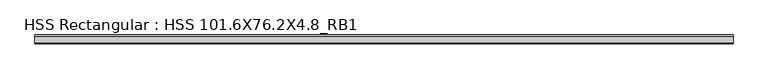
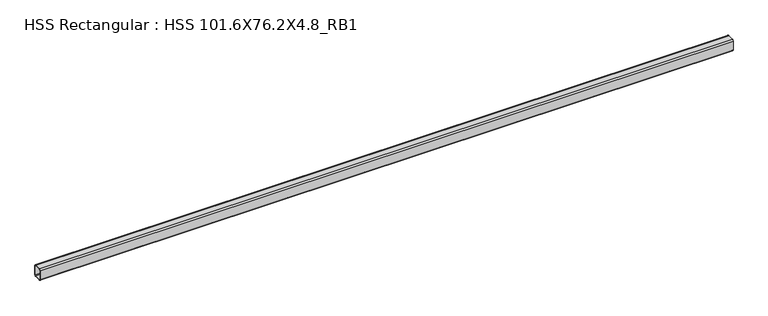
"""IFC4 building model written with IfcOpenShell, lengths in millimetres: beam geometry, HSS Rectangular : HSS 101.6X76.2X4.8_RB1."""

from ifc_helpers import new_model, si_unit, point, frame, frame_2d, origin, place, context, project, spatial, polyline, circle_curve, trimmed, segment, composite_curve, outline, extrude, source, transform, mapped, element, save


def hss_rectangular_hss_101_6x76_2x4_8_rb1_d5c3e1c3(model_context):
    return source(origin(), model_context, "Body", "SweptSolid", [
        extrude(outline(composite_curve([segment(polyline([(38.1, 41.275), (38.1, -41.275)]), True, "CONTINUOUS"), segment(trimmed(circle_curve(frame_2d((28.575, -41.275)), 9.525), [point((38.1, -41.275))], [point((28.575, -50.8))], False, "CARTESIAN"), True, "CONTINUOUS"), segment(polyline([(28.575, -50.8), (-28.575, -50.8)]), True, "CONTINUOUS"), segment(trimmed(circle_curve(frame_2d((-28.575, -41.275)), 9.525), [point((-28.575, -50.8))], [point((-38.1, -41.275))], False, "CARTESIAN"), True, "CONTINUOUS"), segment(polyline([(-38.1, -41.275), (-38.1, 41.275)]), True, "CONTINUOUS"), segment(trimmed(circle_curve(frame_2d((-28.575, 41.275)), 9.525), [point((-38.1, 41.275))], [point((-28.575, 50.8))], False, "CARTESIAN"), True, "CONTINUOUS"), segment(polyline([(-28.575, 50.8), (28.575, 50.8)]), True, "CONTINUOUS"), segment(trimmed(circle_curve(frame_2d((28.575, 41.275)), 9.525), [point((28.575, 50.8))], [point((38.1, 41.275))], False, "CARTESIAN"), True, "CONTINUOUS")], self_intersect=False), holes=[composite_curve([segment(trimmed(circle_curve(frame_2d((-28.575, 41.275)), 4.7625), [point((-28.575, 46.0375))], [point((-33.3375, 41.275))], True, "CARTESIAN"), True, "CONTINUOUS"), segment(polyline([(-33.3375, 41.275), (-33.3375, -41.275)]), True, "CONTINUOUS"), segment(trimmed(circle_curve(frame_2d((-28.575, -41.275)), 4.7625), [point((-33.3375, -41.275))], [point((-28.575, -46.0375))], True, "CARTESIAN"), True, "CONTINUOUS"), segment(polyline([(-28.575, -46.0375), (28.575, -46.0375)]), True, "CONTINUOUS"), segment(trimmed(circle_curve(frame_2d((28.575, -41.275)), 4.7625), [point((28.575, -46.0375))], [point((33.3375, -41.275))], True, "CARTESIAN"), True, "CONTINUOUS"), segment(polyline([(33.3375, -41.275), (33.3375, 41.275)]), True, "CONTINUOUS"), segment(trimmed(circle_curve(frame_2d((28.575, 41.275)), 4.7625), [point((33.3375, 41.275))], [point((28.575, 46.0375))], True, "CARTESIAN"), True, "CONTINUOUS"), segment(polyline([(28.575, 46.0375), (-28.575, 46.0375)]), True, "CONTINUOUS")], self_intersect=False)]), frame((-7509.4611928, 0.0, 0.0), z_axis=(1.0, 0.0, 0.0), x_axis=(0.0, 1.0, 0.0)), (0.0, 0.0, 1.0), 5981.472779),
    ])


if __name__ == "__main__":
    model = new_model("IFC4")
    model_context = context("Model", 3, world=origin())
    ifc_project = project(units=[si_unit("LENGTHUNIT", "METRE", prefix="MILLI")], contexts=[model_context])
    site = spatial("IfcSite", under=ifc_project)
    building = spatial("IfcBuilding", under=site)
    placement = place(None, origin())
    hss_rectangular_hss_101_6x76_2x4_8_rb1_shape = hss_rectangular_hss_101_6x76_2x4_8_rb1_d5c3e1c3(model_context)
    element("IfcBeam", 1, ObjectType="HSS Rectangular : HSS 101.6X76.2X4.8_RB1", at=placement, inside=building, context=model_context, shape_type="MappedRepresentation", body=[
        mapped(hss_rectangular_hss_101_6x76_2x4_8_rb1_shape, transform((0.0, 0.0, 0.0), x_axis=(1.0, 0.0, 0.0), y_axis=(0.0, 1.0, 0.0), z_axis=(0.0, 0.0, 1.0))),
    ])
    save(model, "model.ifc")

# Revit data of these elements
# Type "HSS Rectangular : HSS 101.6X76.2X4.8_RB1"
#   Section Name Key = "HSS 4X3X3/16"
#   Assembly Code = "B10"
#   Width = 7.62 cm
#   Wall Nominal Thickness = 0.4763 cm
#   Wall Design Thickness = 0.442 cm
#   Torsional Moment of Inertia = 260.561 cm⁴
#   Torsional Modulus = 61.2876 cm³
#   Section Area = 14.4516 cm²
#   Plastic Modulus weak axis = 40.3122 cm³
#   Plastic Modulus strong axis = 49.1612 cm³
#   Perimeter = 0.881482 m²/m
#   Outer Fillet = 0.9525 cm
#   Nominal Weight = 12.1285 kgf/m
#   Moment of Inertia weak axis = 131.529 cm⁴
#   Moment of Inertia strong axis = 205.202 cm⁴
#   Inner Fillet = 0.4763 cm
#   Height = 10.16 cm
#   Elastic Modulus weak axis = 34.4128 cm³
#   Elastic Modulus strong axis = 40.476 cm³
#   Centroid Vertical = 5.08 cm
#   Centroid Horizontal = 3.81 cm
#   Length [instance default] = 1524 mm
#   Structural Material [instance default] = Steel ASTM A500, Grade B, Rectangular and Square
#   Principal Axes Angle = 0
# Element 1 (IfcBeam, "HSS Rectangular : HSS 101.6X76.2X4.8_RB1")
#   Structural Material = Steel ASTM A992
#   Materials on its faces: "Steel ASTM A992"
# Materials
#   "Steel ASTM A500, Grade B, Rectangular and Square": class "Metal", colour RGB 199 199 199, transparency 0, Description = "Carbon steel", Cost = 0
#   "Steel ASTM A992": class "Metal", colour RGB 199 199 199, transparency 0, Description = "Structural steel 50ksi", Cost = 0
